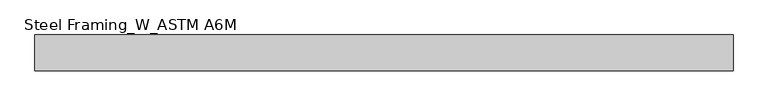
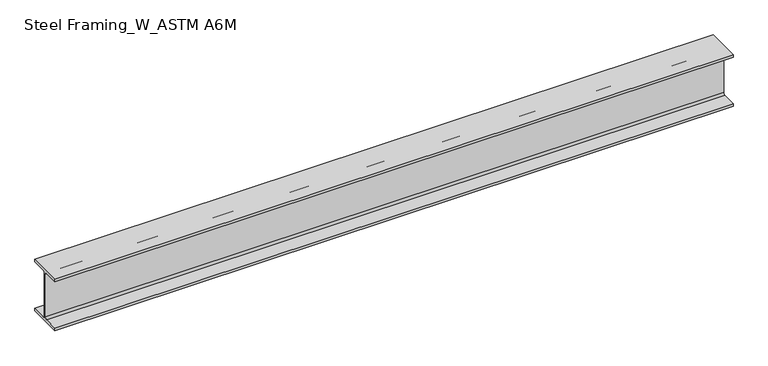
"""IFC4 building model written with IfcOpenShell, lengths in millimetres: beam geometry, Steel Framing_W_ASTM A6M : H_SB_AR_S02_W200x31.3_B6."""

from ifc_helpers import new_model, si_unit, point, frame, frame_2d, origin, place, context, project, spatial, polyline, circle_curve, trimmed, segment, composite_curve, outline, extrude, source, transform, mapped, element, save


def steel_framing_w_astm_a6m_04ed26ec(model_context):
    return source(origin(), model_context, "Body", "SweptSolid", [
        extrude(outline(composite_curve([segment(polyline([(67.0, -94.8), (67.0, -105.0), (-67.0, -105.0), (-67.0, -94.8), (-10.775, -94.8)]), True, "CONTINUOUS"), segment(trimmed(circle_curve(frame_2d((-10.775, -87.2)), 7.6), [point((-10.775, -94.8))], [point((-3.175, -87.2))], True, "CARTESIAN"), True, "CONTINUOUS"), segment(polyline([(-3.175, -87.2), (-3.175, 87.2)]), True, "CONTINUOUS"), segment(trimmed(circle_curve(frame_2d((-10.775, 87.2)), 7.6), [point((-3.175, 87.2))], [point((-10.775, 94.8))], True, "CARTESIAN"), True, "CONTINUOUS"), segment(polyline([(-10.775, 94.8), (-67.0, 94.8), (-67.0, 105.0), (67.0, 105.0), (67.0, 94.8), (10.775, 94.8)]), True, "CONTINUOUS"), segment(trimmed(circle_curve(frame_2d((10.775, 87.2)), 7.6), [point((10.775, 94.8))], [point((3.175, 87.2))], True, "CARTESIAN"), True, "CONTINUOUS"), segment(polyline([(3.175, 87.2), (3.175, -87.2)]), True, "CONTINUOUS"), segment(trimmed(circle_curve(frame_2d((10.775, -87.2)), 7.6), [point((3.175, -87.2))], [point((10.775, -94.8))], True, "CARTESIAN"), True, "CONTINUOUS"), segment(polyline([(10.775, -94.8), (67.0, -94.8)]), True, "CONTINUOUS")], self_intersect=False)), frame((-1346.3, 0.0, 0.0), z_axis=(1.0, 0.0, 0.0), x_axis=(0.0, 1.0, 0.0)), (0.0, 0.0, 1.0), 2620.8),
    ])


if __name__ == "__main__":
    model = new_model("IFC4")
    model_context = context("Model", 3, world=origin())
    ifc_project = project(units=[si_unit("LENGTHUNIT", "METRE", prefix="MILLI")], contexts=[model_context])
    site = spatial("IfcSite", under=ifc_project)
    building = spatial("IfcBuilding", under=site)
    placement = place(None, origin())
    steel_framing_w_astm_a6m_shape = steel_framing_w_astm_a6m_04ed26ec(model_context)
    element("IfcBeam", 1, ObjectType="Steel Framing_W_ASTM A6M : H_SB_AR_S02_W200x31.3_B6", at=placement, inside=building, context=model_context, shape_type="MappedRepresentation", body=[
        mapped(steel_framing_w_astm_a6m_shape, transform((0.0, 0.0, 0.0), x_axis=(1.0, 0.0, 0.0), y_axis=(0.0, 1.0, 0.0), z_axis=(0.0, 0.0, 1.0))),
    ])
    save(model, "model.ifc")

# Revit data of these elements
# Type "Steel Framing_W_ASTM A6M : H_SB_AR_S02_W200x31.3_B6"
#   Type Mark = "B6"
#   Section Name Key = "W8x21"
#   Width = 13.4 cm
#   Web Thickness = 0.635 cm
#   Web Fillet = 0.76 cm
#   Warping Constant = 40800.0 cm⁶
#   Torsional Moment of Inertia = 11.70 cm⁴
#   Section Area = 39.7 cm²
#   Plastic Modulus weak axis = 93.2 cm³
#   Plastic Modulus strong axis = 334.0 cm³
#   Perimeter = 0.93 m²/m
#   Nominal Weight = 31.30 kgf/m
#   Moment of Inertia weak axis = 407.00 cm⁴
#   Moment of Inertia strong axis = 3130.00 cm⁴
#   Height = 21.0 cm
#   Flange Thickness = 1.02 cm
#   Elastic Modulus weak axis = 60.8 cm³
#   Elastic Modulus strong axis = 298.0 cm³
#   Centroid Vertical = 10.5 cm
#   Centroid Horizontal = 6.7 cm
#   Length [instance default] = 1500 mm
#   Structural Material [instance default] = Steel, 45-345
#   Bolt Spacing = 0
#   Assembly Code = ""
# Element 1 (IfcBeam, "Steel Framing_W_ASTM A6M : H_SB_AR_S02_W200x31.3_B6")
#   Materials on its faces: "Steel, 45-345"
# Materials
#   "Steel, 45-345": class "Metal", colour RGB 189 187 185, transparency 0, Description = "Steel 345 MPa", Cost = 0
